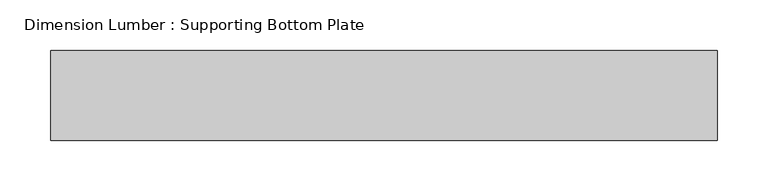
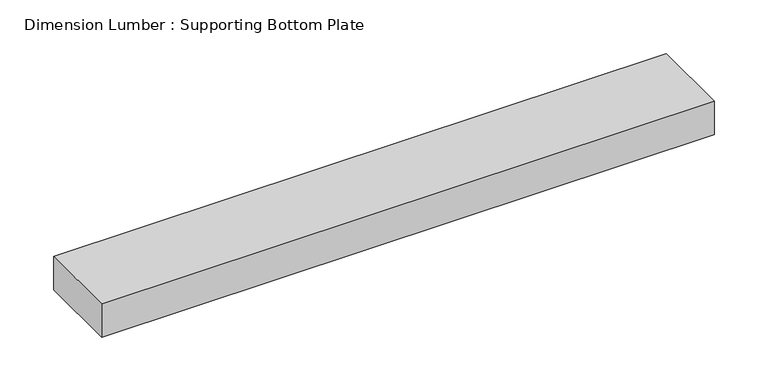
"""IFC4 building model written with IfcOpenShell, lengths in millimetres: beam geometry, Dimension Lumber : Supporting Bottom Plate."""

from ifc_helpers import new_model, si_unit, frame, origin, place, context, project, spatial, polyline, outline, extrude, source, transform, mapped, element, save


def dimension_lumber_supporting_bottom_plate_e3733361(model_context):
    return source(origin(), model_context, "Body", "SweptSolid", [
        extrude(outline(polyline([(328.9051334, 44.45), (328.9051334, -44.45), (-328.9051334, -44.45), (-328.9051334, 44.45), (328.9051334, 44.45)])), frame((0.0, 0.0, -19.05), z_axis=(0.0, 0.0, 1.0), x_axis=(1.0, 0.0, 0.0)), (0.0, 0.0, 1.0), 38.1),
    ])


if __name__ == "__main__":
    model = new_model("IFC4")
    model_context = context("Model", 3, world=origin())
    ifc_project = project(units=[si_unit("LENGTHUNIT", "METRE", prefix="MILLI")], contexts=[model_context])
    site = spatial("IfcSite", under=ifc_project)
    building = spatial("IfcBuilding", under=site)
    placement = place(None, origin())
    dimension_lumber_supporting_bottom_plate_shape = dimension_lumber_supporting_bottom_plate_e3733361(model_context)
    element("IfcBeam", 1, ObjectType="Dimension Lumber : Supporting Bottom Plate", at=placement, inside=building, context=model_context, shape_type="MappedRepresentation", body=[
        mapped(dimension_lumber_supporting_bottom_plate_shape, transform((0.0, 0.0, 0.0), x_axis=(1.0, 0.0, 0.0), y_axis=(0.0, 1.0, 0.0), z_axis=(0.0, 0.0, 1.0))),
    ])
    save(model, "model.ifc")

# Revit data of these elements
# Type "Dimension Lumber : Supporting Bottom Plate"
#   Assembly Code = "B10"
#   A = 0.0364583 SF
#   Length [instance default] = 5' - 0"
#   b = 0' - 3 1/2"
#   d = 0' - 1 1/2"
#   Structural Material [instance default] = Softwood, Lumber
# Element 1 (IfcBeam, "Dimension Lumber : Supporting Bottom Plate")
#   Structural Material = Douglas Fir #2
#   Materials on its faces: "Douglas Fir #2"
# Materials
#   "Softwood, Lumber": class "Wood", colour RGB 223 192 134, transparency 0, Description = "Pinus Echinata", Cost = 0
#   "Douglas Fir #2": class "Wood", colour RGB 223 192 134, transparency 0, Description = "Pinus Echinata", Cost = 0
